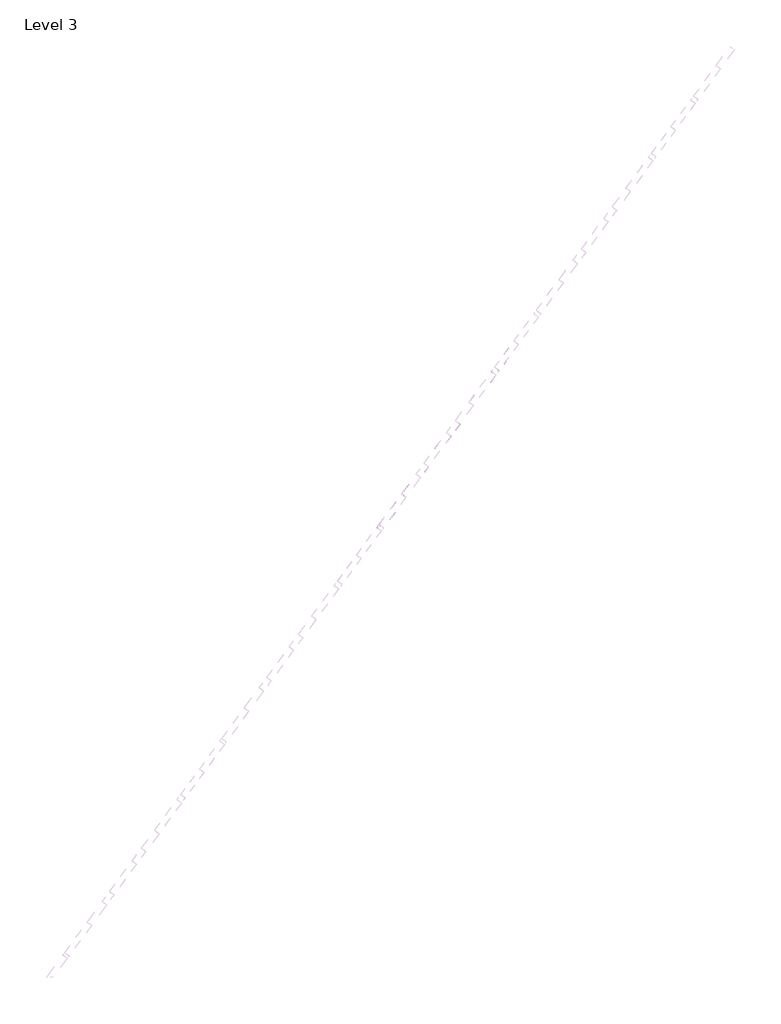
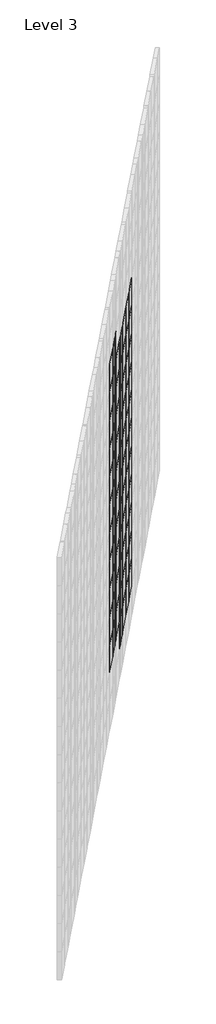
# One storey, part 7 of 9: 120 plates.
"""IFC4 building model written with IfcOpenShell, lengths in millimetres."""

import ifcopenshell
import ifcopenshell.guid

model = None  # the IFC model being written
_history = None  # IfcOwnerHistory: only IFC2X3 demands one
_inside = {}  # id of a spatial element -> (the spatial element, [elements in it])
_under = {}  # id of a project, library or spatial element -> (it, [spatial elements below it])
_declared = {}  # id of a project -> (the project, [libraries it declares])
_typed = {}  # id of a type object -> (the type object, [elements of that type])
_made_of = {}  # id of a material, layer set ... -> (it, [elements and type objects made of it])


def new_model(schema):
    """Start an empty IFC model of exactly this schema.

    Asked for "IFC4X3", IfcOpenShell would pick the latest addendum, in which some entities
    have other attributes; the version numbers below select the first issue.
    IFC2X3 requires an IfcOwnerHistory on every rooted entity: one is made here for all.
    """
    global model, _history
    if schema == "IFC4X3":
        model = ifcopenshell.file(schema_version=(4, 3, 0, 0))
    else:
        model = ifcopenshell.file(schema=schema)
    _inside.clear()
    _under.clear()
    _declared.clear()
    _typed.clear()
    _made_of.clear()
    _history = None
    if model.schema == "IFC2X3":
        org = make("IfcOrganization", Name="unknown")
        user = make(
            "IfcPersonAndOrganization",
            ThePerson=make("IfcPerson", FamilyName="unknown"),
            TheOrganization=org,
        )
        app = make(
            "IfcApplication",
            ApplicationDeveloper=org,
            Version="unknown",
            ApplicationFullName="unknown",
            ApplicationIdentifier="unknown",
        )
        _history = make(
            "IfcOwnerHistory",
            OwningUser=user,
            OwningApplication=app,
            ChangeAction="ADDED",
            CreationDate=0,
        )
    return model


def make(cls, **values):
    """One entity of the class cls with the attributes given. An attribute that is None is left unset."""
    return model.create_entity(
        cls, **{name: value for name, value in values.items() if value is not None}
    )


def rooted(cls, **values):
    """An entity with a GlobalId (a new one), such as an element, a storey or a relation."""
    return make(cls, GlobalId=ifcopenshell.guid.new(), OwnerHistory=_history, **values)


def si_unit(unit_type, name, prefix=None):
    """IfcSIUnit, for example si_unit("LENGTHUNIT", "METRE", prefix="MILLI")."""
    return make("IfcSIUnit", UnitType=unit_type, Prefix=prefix, Name=name)


def assignment(units):
    """IfcUnitAssignment: the units of a project."""
    return None if units is None else make("IfcUnitAssignment", Units=units)


def point(xyz):
    """IfcCartesianPoint."""
    return None if xyz is None else make("IfcCartesianPoint", Coordinates=xyz)


def direction(xyz):
    """IfcDirection."""
    return None if xyz is None else make("IfcDirection", DirectionRatios=xyz)


def frame(location, z_axis=None, x_axis=None):
    """IfcAxis2Placement3D, a coordinate frame: its origin and axes. An axis left out is left unset."""
    return make(
        "IfcAxis2Placement3D",
        Location=point(location),
        Axis=direction(z_axis),
        RefDirection=direction(x_axis),
    )


def origin():
    """The frame at (0, 0, 0) with its axes left unset."""
    return frame((0.0, 0.0, 0.0))


def origin_with_axes():
    """The frame at (0, 0, 0) with the z axis (0, 0, 1) and the x axis (1, 0, 0) written out."""
    return frame((0.0, 0.0, 0.0), z_axis=(0.0, 0.0, 1.0), x_axis=(1.0, 0.0, 0.0))


def place(relative_to, where):
    """IfcLocalPlacement: puts the frame where relative to a parent placement (None: the world)."""
    return make(
        "IfcLocalPlacement", PlacementRelTo=relative_to, RelativePlacement=where
    )


def context(
    kind, dimensions, precision=None, world=None, true_north=None, identifier=None
):
    """IfcGeometricRepresentationContext, for example the 3D "Model" context."""
    return make(
        "IfcGeometricRepresentationContext",
        ContextIdentifier=identifier,
        ContextType=kind,
        CoordinateSpaceDimension=dimensions,
        Precision=precision,
        WorldCoordinateSystem=world,
        TrueNorth=true_north,
    )


def project(units=None, contexts=None):
    """IfcProject with its units and contexts."""
    return rooted(
        "IfcProject",
        Name="project",
        RepresentationContexts=contexts,
        UnitsInContext=assignment(units),
    )


def spatial(cls, under=None, at=None, **own):
    """A site, building, storey or space (cls), placed at a placement, below another one or the project."""
    s = rooted(cls, ObjectPlacement=at, **own)
    if under is not None:
        _under.setdefault(under.id(), (under, []))[1].append(s)
    return s


def polyline(points):
    """IfcPolyline through the points."""
    return make("IfcPolyline", Points=[point(p) for p in points])


def outline(outer, holes=None, kind="AREA"):
    """IfcArbitraryClosedProfileDef: a profile drawn as a closed curve; with holes, ...WithVoids."""
    if holes is None:
        return make("IfcArbitraryClosedProfileDef", ProfileType=kind, OuterCurve=outer)
    return make(
        "IfcArbitraryProfileDefWithVoids",
        ProfileType=kind,
        OuterCurve=outer,
        InnerCurves=holes,
    )


def extrude(swept, where, along, depth):
    """IfcExtrudedAreaSolid: the profile swept, set in the frame where, extruded along a direction by depth."""
    return make(
        "IfcExtrudedAreaSolid",
        SweptArea=swept,
        Position=where,
        ExtrudedDirection=direction(along),
        Depth=depth,
    )


def shape(context_of_items, identifier, shape_type, items):
    """IfcShapeRepresentation: the items that make up one representation, for example the "Body"."""
    return make(
        "IfcShapeRepresentation",
        ContextOfItems=context_of_items,
        RepresentationIdentifier=identifier,
        RepresentationType=shape_type,
        Items=items,
    )


def source(mapping_origin, context_of_items, identifier, shape_type, items):
    """IfcRepresentationMap: a shape defined once, which mapped items show again and again."""
    return make(
        "IfcRepresentationMap",
        MappingOrigin=mapping_origin,
        MappedRepresentation=shape(context_of_items, identifier, shape_type, items),
    )


def transform(
    local_origin,
    x_axis=None,
    y_axis=None,
    z_axis=None,
    scale=None,
    scale2=None,
    scale3=None,
    uniform=True,
):
    """IfcCartesianTransformationOperator3D, or its non-uniform kind. x_axis, y_axis, z_axis: its Axis1, 2, 3."""
    if uniform:
        return make(
            "IfcCartesianTransformationOperator3D",
            Axis1=direction(x_axis),
            Axis2=direction(y_axis),
            LocalOrigin=point(local_origin),
            Scale=scale,
            Axis3=direction(z_axis),
        )
    return make(
        "IfcCartesianTransformationOperator3DnonUniform",
        Axis1=direction(x_axis),
        Axis2=direction(y_axis),
        LocalOrigin=point(local_origin),
        Scale=scale,
        Axis3=direction(z_axis),
        Scale2=scale2,
        Scale3=scale3,
    )


def mapped(mapping_source, mapping_target):
    """IfcMappedItem: shows the shape of a source again, moved by a transform."""
    return make(
        "IfcMappedItem", MappingSource=mapping_source, MappingTarget=mapping_target
    )


def made_of(thing, what):
    """Note that an element or type object is made of a material, layer set ...; save() writes the relation."""
    if what is not None:
        _made_of.setdefault(what.id(), (what, []))[1].append(thing)
    return thing


def element(
    cls,
    number,
    at=None,
    inside=None,
    cuts=None,
    type_object=None,
    material=None,
    context=None,
    identifier="Body",
    shape_type=None,
    held_by="IfcProductDefinitionShape",
    body=None,
    shapes=None,
    **own,
):
    """One element of the class cls, such as IfcWall. Its Tag is "e" and its number.

    at: its placement. inside: the storey or other place that contains it. cuts: it is an
    opening in that element (IfcRelVoidsElement). A single representation is given by context,
    identifier, shape_type and body (its items); several are given by shapes. held_by: the class
    of the entity that holds the representations. save() writes the other relations.
    """
    e = rooted(cls, Tag="e%d" % number, ObjectPlacement=at, **own)
    if body is not None:
        shapes = [shape(context, identifier, shape_type, body)]
    if shapes is not None:
        e.Representation = make(held_by, Representations=shapes)
    if inside is not None:
        _inside.setdefault(inside.id(), (inside, []))[1].append(e)
    if cuts is not None:
        rooted(
            "IfcRelVoidsElement", RelatingBuildingElement=cuts, RelatedOpeningElement=e
        )
    if type_object is not None:
        _typed.setdefault(type_object.id(), (type_object, []))[1].append(e)
    return made_of(e, material)


def aggregate(whole, parts):
    """IfcRelAggregates: a whole, such as a stair, and the parts it consists of."""
    return rooted("IfcRelAggregates", RelatingObject=whole, RelatedObjects=parts)


def save(model, path):
    """Write the relations noted so far, then the file.

    IfcRelAggregates (storeys below a building ...), IfcRelContainedInSpatialStructure (elements
    in a storey), IfcRelDefinesByType, IfcRelAssociatesMaterial and IfcRelDeclares: one each for
    every whole, place, type object, material and project.
    """
    for whole, parts in _under.values():
        aggregate(whole, parts)
    for where, things in _inside.values():
        rooted(
            "IfcRelContainedInSpatialStructure",
            RelatedElements=things,
            RelatingStructure=where,
        )
    for kind, things in _typed.values():
        rooted("IfcRelDefinesByType", RelatedObjects=things, RelatingType=kind)
    for what, things in _made_of.values():
        rooted("IfcRelAssociatesMaterial", RelatedObjects=things, RelatingMaterial=what)
    for by, libraries in _declared.values():
        rooted("IfcRelDeclares", RelatingContext=by, RelatedDefinitions=libraries)
    model.write(path)


def system_panel_glazed_b646d57f(model_context):
    return source(origin(), model_context, "Body", "SweptSolid", [
        extrude(outline(polyline([(8.5363468, 24.5), (-8.5363468, 24.5), (-8.5363468, 49.5), (8.5363468, 49.5), (8.5363468, 24.5)])), origin_with_axes(), (0.0, 0.0, 1.0), 200.0),
    ])


def system_panel_glazed_944c5575(model_context):
    return source(origin(), model_context, "Body", "SweptSolid", [
        extrude(outline(polyline([(30.0531077, 24.5), (-30.0531077, 24.5), (-30.0531077, 49.5), (30.0531077, 49.5), (30.0531077, 24.5)])), origin_with_axes(), (0.0, 0.0, 1.0), 200.0),
    ])


def system_panel_glazed_4b393385(model_context):
    return source(origin(), model_context, "Body", "SweptSolid", [
        extrude(outline(polyline([(51.5698685, 24.5), (-51.5698685, 24.5), (-51.5698685, 49.5), (51.5698685, 49.5), (51.5698685, 24.5)])), origin_with_axes(), (0.0, 0.0, 1.0), 200.0),
    ])


def system_panel_glazed_44cc28f0(model_context):
    return source(origin(), model_context, "Body", "SweptSolid", [
        extrude(outline(polyline([(73.0866293, 24.5), (-73.0866293, 24.5), (-73.0866293, 49.5), (73.0866293, 49.5), (73.0866293, 24.5)])), origin_with_axes(), (0.0, 0.0, 1.0), 200.0),
    ])


def system_panel_glazed_1ea8d406(model_context):
    return source(origin(), model_context, "Body", "SweptSolid", [
        extrude(outline(polyline([(85.0, 24.5), (-85.0, 24.5), (-85.0, 49.5), (85.0, 49.5), (85.0, 24.5)])), origin_with_axes(), (0.0, 0.0, 1.0), 200.0),
    ])


def system_panel_glazed_a6cffc9f(model_context):
    return source(origin(), model_context, "Body", "SweptSolid", [
        extrude(outline(polyline([(54.9468923, 24.5), (-54.9468923, 24.5), (-54.9468923, 49.5), (54.9468923, 49.5), (54.9468923, 24.5)])), origin_with_axes(), (0.0, 0.0, 1.0), 200.0),
    ])


def system_panel_glazed_52e3984b(model_context):
    return source(origin(), model_context, "Body", "SweptSolid", [
        extrude(outline(polyline([(33.4301315, 24.5), (-33.4301315, 24.5), (-33.4301315, 49.5), (33.4301315, 49.5), (33.4301315, 24.5)])), origin_with_axes(), (0.0, 0.0, 1.0), 200.0),
    ])


def system_panel_glazed_aeb916ba(model_context):
    return source(origin(), model_context, "Body", "SweptSolid", [
        extrude(outline(polyline([(11.9133707, 24.5), (-11.9133707, 24.5), (-11.9133707, 49.5), (11.9133707, 49.5), (11.9133707, 24.5)])), origin_with_axes(), (0.0, 0.0, 1.0), 200.0),
    ])


def system_panel_glazed_a3c9f580(model_context):
    return source(origin(), model_context, "Body", "SweptSolid", [
        extrude(outline(polyline([(75.3966098, 24.5), (-75.3966098, 24.5), (-75.3966098, 49.5), (75.3966098, 49.5), (75.3966098, 24.5)])), origin_with_axes(), (0.0, 0.0, 1.0), 200.0),
    ])


model = new_model("IFC4")

# Units and contexts
model_context = context("Model", 3, world=origin())
ifc_project = project(units=[si_unit("LENGTHUNIT", "METRE", prefix="MILLI")], contexts=[model_context])

# Site, building, storey
site = spatial("IfcSite", under=ifc_project)
building = spatial("IfcBuilding", under=site)
storey = spatial("IfcBuildingStorey", under=building, Name="Level 3", Elevation=22950.0)

# Plates
placement = place(None, origin())
system_panel_glazed_shape = system_panel_glazed_b646d57f(model_context)
element("IfcPlate", 1, ObjectType="System Panel : Glazed", at=placement, inside=storey, context=model_context, shape_type="MappedRepresentation", body=[
    mapped(system_panel_glazed_shape, transform((-31872.965562, 30068.174428, 35500.0), x_axis=(0.5920548138930122, 0.8058976965757569, 0.0), y_axis=(-0.8058976965757569, 0.5920548138930122, 0.0), z_axis=(0.0, 0.0, 1.0))),
])
element("IfcPlate", 2, ObjectType="System Panel : Glazed", at=placement, inside=storey, context=model_context, shape_type="MappedRepresentation", body=[
    mapped(system_panel_glazed_shape, transform((-31872.965562, 30068.174428, 35700.0), x_axis=(0.5920548138930122, 0.8058976965757569, 0.0), y_axis=(-0.8058976965757569, 0.5920548138930122, 0.0), z_axis=(0.0, 0.0, 1.0))),
])
element("IfcPlate", 3, ObjectType="System Panel : Glazed", at=placement, inside=storey, context=model_context, shape_type="MappedRepresentation", body=[
    mapped(system_panel_glazed_shape, transform((-31872.965562, 30068.174428, 35900.0), x_axis=(0.5920548138930122, 0.8058976965757569, 0.0), y_axis=(-0.8058976965757569, 0.5920548138930122, 0.0), z_axis=(0.0, 0.0, 1.0))),
])
element("IfcPlate", 4, ObjectType="System Panel : Glazed", at=placement, inside=storey, context=model_context, shape_type="MappedRepresentation", body=[
    mapped(system_panel_glazed_shape, transform((-31872.965562, 30068.174428, 36100.0), x_axis=(0.5920548138930122, 0.8058976965757569, 0.0), y_axis=(-0.8058976965757569, 0.5920548138930122, 0.0), z_axis=(0.0, 0.0, 1.0))),
])
element("IfcPlate", 5, ObjectType="System Panel : Glazed", at=placement, inside=storey, context=model_context, shape_type="MappedRepresentation", body=[
    mapped(system_panel_glazed_shape, transform((-31872.965562, 30068.174428, 36300.0), x_axis=(0.5920548138930122, 0.8058976965757569, 0.0), y_axis=(-0.8058976965757569, 0.5920548138930122, 0.0), z_axis=(0.0, 0.0, 1.0))),
])
element("IfcPlate", 6, ObjectType="System Panel : Glazed", at=placement, inside=storey, context=model_context, shape_type="MappedRepresentation", body=[
    mapped(system_panel_glazed_shape, transform((-31872.965562, 30068.174428, 36500.0), x_axis=(0.5920548138930122, 0.8058976965757569, 0.0), y_axis=(-0.8058976965757569, 0.5920548138930122, 0.0), z_axis=(0.0, 0.0, 1.0))),
])
element("IfcPlate", 7, ObjectType="System Panel : Glazed", at=placement, inside=storey, context=model_context, shape_type="MappedRepresentation", body=[
    mapped(system_panel_glazed_shape, transform((-31872.965562, 30068.174428, 36700.0), x_axis=(0.5920548138930122, 0.8058976965757569, 0.0), y_axis=(-0.8058976965757569, 0.5920548138930122, 0.0), z_axis=(0.0, 0.0, 1.0))),
])
element("IfcPlate", 8, ObjectType="System Panel : Glazed", at=placement, inside=storey, context=model_context, shape_type="MappedRepresentation", body=[
    mapped(system_panel_glazed_shape, transform((-31872.965562, 30068.174428, 36900.0), x_axis=(0.5920548138930122, 0.8058976965757569, 0.0), y_axis=(-0.8058976965757569, 0.5920548138930122, 0.0), z_axis=(0.0, 0.0, 1.0))),
])
element("IfcPlate", 9, ObjectType="System Panel : Glazed", at=placement, inside=storey, context=model_context, shape_type="MappedRepresentation", body=[
    mapped(system_panel_glazed_shape, transform((-31872.965562, 30068.174428, 37100.0), x_axis=(0.5920548138930122, 0.8058976965757569, 0.0), y_axis=(-0.8058976965757569, 0.5920548138930122, 0.0), z_axis=(0.0, 0.0, 1.0))),
])
element("IfcPlate", 10, ObjectType="System Panel : Glazed", at=placement, inside=storey, context=model_context, shape_type="MappedRepresentation", body=[
    mapped(system_panel_glazed_shape, transform((-31872.965562, 30068.174428, 37300.0), x_axis=(0.5920548138930122, 0.8058976965757569, 0.0), y_axis=(-0.8058976965757569, 0.5920548138930122, 0.0), z_axis=(0.0, 0.0, 1.0))),
])
element("IfcPlate", 11, ObjectType="System Panel : Glazed", at=placement, inside=storey, context=model_context, shape_type="MappedRepresentation", body=[
    mapped(system_panel_glazed_shape, transform((-31872.965562, 30068.174428, 37500.0), x_axis=(0.5920548138930122, 0.8058976965757569, 0.0), y_axis=(-0.8058976965757569, 0.5920548138930122, 0.0), z_axis=(0.0, 0.0, 1.0))),
])
system_panel_glazed_2_shape = system_panel_glazed_944c5575(model_context)
element("IfcPlate", 12, ObjectType="System Panel : Glazed", at=placement, inside=storey, context=model_context, shape_type="MappedRepresentation", body=[
    mapped(system_panel_glazed_2_shape, transform((-31684.4060271, 30324.8393368, 35500.0), x_axis=(0.5920548138930122, 0.8058976965757569, 0.0), y_axis=(-0.8058976965757569, 0.5920548138930122, 0.0), z_axis=(0.0, 0.0, 1.0))),
])
element("IfcPlate", 13, ObjectType="System Panel : Glazed", at=placement, inside=storey, context=model_context, shape_type="MappedRepresentation", body=[
    mapped(system_panel_glazed_2_shape, transform((-31684.4060271, 30324.8393368, 35700.0), x_axis=(0.5920548138930122, 0.8058976965757569, 0.0), y_axis=(-0.8058976965757569, 0.5920548138930122, 0.0), z_axis=(0.0, 0.0, 1.0))),
])
element("IfcPlate", 14, ObjectType="System Panel : Glazed", at=placement, inside=storey, context=model_context, shape_type="MappedRepresentation", body=[
    mapped(system_panel_glazed_2_shape, transform((-31684.4060271, 30324.8393368, 35900.0), x_axis=(0.5920548138930122, 0.8058976965757569, 0.0), y_axis=(-0.8058976965757569, 0.5920548138930122, 0.0), z_axis=(0.0, 0.0, 1.0))),
])
element("IfcPlate", 15, ObjectType="System Panel : Glazed", at=placement, inside=storey, context=model_context, shape_type="MappedRepresentation", body=[
    mapped(system_panel_glazed_2_shape, transform((-31684.4060271, 30324.8393368, 36100.0), x_axis=(0.5920548138930122, 0.8058976965757569, 0.0), y_axis=(-0.8058976965757569, 0.5920548138930122, 0.0), z_axis=(0.0, 0.0, 1.0))),
])
element("IfcPlate", 16, ObjectType="System Panel : Glazed", at=placement, inside=storey, context=model_context, shape_type="MappedRepresentation", body=[
    mapped(system_panel_glazed_2_shape, transform((-31684.4060271, 30324.8393368, 36300.0), x_axis=(0.5920548138930122, 0.8058976965757569, 0.0), y_axis=(-0.8058976965757569, 0.5920548138930122, 0.0), z_axis=(0.0, 0.0, 1.0))),
])
element("IfcPlate", 17, ObjectType="System Panel : Glazed", at=placement, inside=storey, context=model_context, shape_type="MappedRepresentation", body=[
    mapped(system_panel_glazed_2_shape, transform((-31684.4060271, 30324.8393368, 36500.0), x_axis=(0.5920548138930122, 0.8058976965757569, 0.0), y_axis=(-0.8058976965757569, 0.5920548138930122, 0.0), z_axis=(0.0, 0.0, 1.0))),
])
element("IfcPlate", 18, ObjectType="System Panel : Glazed", at=placement, inside=storey, context=model_context, shape_type="MappedRepresentation", body=[
    mapped(system_panel_glazed_2_shape, transform((-31684.4060271, 30324.8393368, 36700.0), x_axis=(0.5920548138930122, 0.8058976965757569, 0.0), y_axis=(-0.8058976965757569, 0.5920548138930122, 0.0), z_axis=(0.0, 0.0, 1.0))),
])
element("IfcPlate", 19, ObjectType="System Panel : Glazed", at=placement, inside=storey, context=model_context, shape_type="MappedRepresentation", body=[
    mapped(system_panel_glazed_2_shape, transform((-31684.4060271, 30324.8393368, 36900.0), x_axis=(0.5920548138930122, 0.8058976965757569, 0.0), y_axis=(-0.8058976965757569, 0.5920548138930122, 0.0), z_axis=(0.0, 0.0, 1.0))),
])
element("IfcPlate", 20, ObjectType="System Panel : Glazed", at=placement, inside=storey, context=model_context, shape_type="MappedRepresentation", body=[
    mapped(system_panel_glazed_2_shape, transform((-31684.4060271, 30324.8393368, 37100.0), x_axis=(0.5920548138930122, 0.8058976965757569, 0.0), y_axis=(-0.8058976965757569, 0.5920548138930122, 0.0), z_axis=(0.0, 0.0, 1.0))),
])
element("IfcPlate", 21, ObjectType="System Panel : Glazed", at=placement, inside=storey, context=model_context, shape_type="MappedRepresentation", body=[
    mapped(system_panel_glazed_2_shape, transform((-31684.4060271, 30324.8393368, 37300.0), x_axis=(0.5920548138930122, 0.8058976965757569, 0.0), y_axis=(-0.8058976965757569, 0.5920548138930122, 0.0), z_axis=(0.0, 0.0, 1.0))),
])
element("IfcPlate", 22, ObjectType="System Panel : Glazed", at=placement, inside=storey, context=model_context, shape_type="MappedRepresentation", body=[
    mapped(system_panel_glazed_2_shape, transform((-31684.4060271, 30324.8393368, 37500.0), x_axis=(0.5920548138930122, 0.8058976965757569, 0.0), y_axis=(-0.8058976965757569, 0.5920548138930122, 0.0), z_axis=(0.0, 0.0, 1.0))),
])
system_panel_glazed_3_shape = system_panel_glazed_4b393385(model_context)
element("IfcPlate", 23, ObjectType="System Panel : Glazed", at=placement, inside=storey, context=model_context, shape_type="MappedRepresentation", body=[
    mapped(system_panel_glazed_3_shape, transform((-31495.8464922, 30581.5042456, 35300.0), x_axis=(0.5920548138930122, 0.8058976965757569, 0.0), y_axis=(-0.8058976965757569, 0.5920548138930122, 0.0), z_axis=(0.0, 0.0, 1.0))),
])
element("IfcPlate", 24, ObjectType="System Panel : Glazed", at=placement, inside=storey, context=model_context, shape_type="MappedRepresentation", body=[
    mapped(system_panel_glazed_3_shape, transform((-31495.8464922, 30581.5042456, 35500.0), x_axis=(0.5920548138930122, 0.8058976965757569, 0.0), y_axis=(-0.8058976965757569, 0.5920548138930122, 0.0), z_axis=(0.0, 0.0, 1.0))),
])
element("IfcPlate", 25, ObjectType="System Panel : Glazed", at=placement, inside=storey, context=model_context, shape_type="MappedRepresentation", body=[
    mapped(system_panel_glazed_3_shape, transform((-31495.8464922, 30581.5042456, 35700.0), x_axis=(0.5920548138930122, 0.8058976965757569, 0.0), y_axis=(-0.8058976965757569, 0.5920548138930122, 0.0), z_axis=(0.0, 0.0, 1.0))),
])
element("IfcPlate", 26, ObjectType="System Panel : Glazed", at=placement, inside=storey, context=model_context, shape_type="MappedRepresentation", body=[
    mapped(system_panel_glazed_3_shape, transform((-31495.8464922, 30581.5042456, 35900.0), x_axis=(0.5920548138930122, 0.8058976965757569, 0.0), y_axis=(-0.8058976965757569, 0.5920548138930122, 0.0), z_axis=(0.0, 0.0, 1.0))),
])
element("IfcPlate", 27, ObjectType="System Panel : Glazed", at=placement, inside=storey, context=model_context, shape_type="MappedRepresentation", body=[
    mapped(system_panel_glazed_3_shape, transform((-31495.8464922, 30581.5042456, 36100.0), x_axis=(0.5920548138930122, 0.8058976965757569, 0.0), y_axis=(-0.8058976965757569, 0.5920548138930122, 0.0), z_axis=(0.0, 0.0, 1.0))),
])
element("IfcPlate", 28, ObjectType="System Panel : Glazed", at=placement, inside=storey, context=model_context, shape_type="MappedRepresentation", body=[
    mapped(system_panel_glazed_3_shape, transform((-31495.8464922, 30581.5042456, 36300.0), x_axis=(0.5920548138930122, 0.8058976965757569, 0.0), y_axis=(-0.8058976965757569, 0.5920548138930122, 0.0), z_axis=(0.0, 0.0, 1.0))),
])
element("IfcPlate", 29, ObjectType="System Panel : Glazed", at=placement, inside=storey, context=model_context, shape_type="MappedRepresentation", body=[
    mapped(system_panel_glazed_3_shape, transform((-31495.8464922, 30581.5042456, 36500.0), x_axis=(0.5920548138930122, 0.8058976965757569, 0.0), y_axis=(-0.8058976965757569, 0.5920548138930122, 0.0), z_axis=(0.0, 0.0, 1.0))),
])
element("IfcPlate", 30, ObjectType="System Panel : Glazed", at=placement, inside=storey, context=model_context, shape_type="MappedRepresentation", body=[
    mapped(system_panel_glazed_3_shape, transform((-31495.8464922, 30581.5042456, 36700.0), x_axis=(0.5920548138930122, 0.8058976965757569, 0.0), y_axis=(-0.8058976965757569, 0.5920548138930122, 0.0), z_axis=(0.0, 0.0, 1.0))),
])
element("IfcPlate", 31, ObjectType="System Panel : Glazed", at=placement, inside=storey, context=model_context, shape_type="MappedRepresentation", body=[
    mapped(system_panel_glazed_3_shape, transform((-31495.8464922, 30581.5042456, 36900.0), x_axis=(0.5920548138930122, 0.8058976965757569, 0.0), y_axis=(-0.8058976965757569, 0.5920548138930122, 0.0), z_axis=(0.0, 0.0, 1.0))),
])
element("IfcPlate", 32, ObjectType="System Panel : Glazed", at=placement, inside=storey, context=model_context, shape_type="MappedRepresentation", body=[
    mapped(system_panel_glazed_3_shape, transform((-31495.8464922, 30581.5042456, 37100.0), x_axis=(0.5920548138930122, 0.8058976965757569, 0.0), y_axis=(-0.8058976965757569, 0.5920548138930122, 0.0), z_axis=(0.0, 0.0, 1.0))),
])
element("IfcPlate", 33, ObjectType="System Panel : Glazed", at=placement, inside=storey, context=model_context, shape_type="MappedRepresentation", body=[
    mapped(system_panel_glazed_3_shape, transform((-31495.8464922, 30581.5042456, 37300.0), x_axis=(0.5920548138930122, 0.8058976965757569, 0.0), y_axis=(-0.8058976965757569, 0.5920548138930122, 0.0), z_axis=(0.0, 0.0, 1.0))),
])
system_panel_glazed_4_shape = system_panel_glazed_44cc28f0(model_context)
element("IfcPlate", 34, ObjectType="System Panel : Glazed", at=placement, inside=storey, context=model_context, shape_type="MappedRepresentation", body=[
    mapped(system_panel_glazed_4_shape, transform((-31307.2869573, 30838.1691545, 35300.0), x_axis=(0.5920548138930122, 0.8058976965757569, 0.0), y_axis=(-0.8058976965757569, 0.5920548138930122, 0.0), z_axis=(0.0, 0.0, 1.0))),
])
element("IfcPlate", 35, ObjectType="System Panel : Glazed", at=placement, inside=storey, context=model_context, shape_type="MappedRepresentation", body=[
    mapped(system_panel_glazed_4_shape, transform((-31307.2869573, 30838.1691545, 35500.0), x_axis=(0.5920548138930122, 0.8058976965757569, 0.0), y_axis=(-0.8058976965757569, 0.5920548138930122, 0.0), z_axis=(0.0, 0.0, 1.0))),
])
element("IfcPlate", 36, ObjectType="System Panel : Glazed", at=placement, inside=storey, context=model_context, shape_type="MappedRepresentation", body=[
    mapped(system_panel_glazed_4_shape, transform((-31307.2869573, 30838.1691545, 35700.0), x_axis=(0.5920548138930122, 0.8058976965757569, 0.0), y_axis=(-0.8058976965757569, 0.5920548138930122, 0.0), z_axis=(0.0, 0.0, 1.0))),
])
element("IfcPlate", 37, ObjectType="System Panel : Glazed", at=placement, inside=storey, context=model_context, shape_type="MappedRepresentation", body=[
    mapped(system_panel_glazed_4_shape, transform((-31307.2869573, 30838.1691545, 35900.0), x_axis=(0.5920548138930122, 0.8058976965757569, 0.0), y_axis=(-0.8058976965757569, 0.5920548138930122, 0.0), z_axis=(0.0, 0.0, 1.0))),
])
element("IfcPlate", 38, ObjectType="System Panel : Glazed", at=placement, inside=storey, context=model_context, shape_type="MappedRepresentation", body=[
    mapped(system_panel_glazed_4_shape, transform((-31307.2869573, 30838.1691545, 36100.0), x_axis=(0.5920548138930122, 0.8058976965757569, 0.0), y_axis=(-0.8058976965757569, 0.5920548138930122, 0.0), z_axis=(0.0, 0.0, 1.0))),
])
element("IfcPlate", 39, ObjectType="System Panel : Glazed", at=placement, inside=storey, context=model_context, shape_type="MappedRepresentation", body=[
    mapped(system_panel_glazed_4_shape, transform((-31307.2869573, 30838.1691545, 36300.0), x_axis=(0.5920548138930122, 0.8058976965757569, 0.0), y_axis=(-0.8058976965757569, 0.5920548138930122, 0.0), z_axis=(0.0, 0.0, 1.0))),
])
element("IfcPlate", 40, ObjectType="System Panel : Glazed", at=placement, inside=storey, context=model_context, shape_type="MappedRepresentation", body=[
    mapped(system_panel_glazed_4_shape, transform((-31307.2869573, 30838.1691545, 36500.0), x_axis=(0.5920548138930122, 0.8058976965757569, 0.0), y_axis=(-0.8058976965757569, 0.5920548138930122, 0.0), z_axis=(0.0, 0.0, 1.0))),
])
element("IfcPlate", 41, ObjectType="System Panel : Glazed", at=placement, inside=storey, context=model_context, shape_type="MappedRepresentation", body=[
    mapped(system_panel_glazed_4_shape, transform((-31307.2869573, 30838.1691545, 36700.0), x_axis=(0.5920548138930122, 0.8058976965757569, 0.0), y_axis=(-0.8058976965757569, 0.5920548138930122, 0.0), z_axis=(0.0, 0.0, 1.0))),
])
element("IfcPlate", 42, ObjectType="System Panel : Glazed", at=placement, inside=storey, context=model_context, shape_type="MappedRepresentation", body=[
    mapped(system_panel_glazed_4_shape, transform((-31307.2869573, 30838.1691545, 36900.0), x_axis=(0.5920548138930122, 0.8058976965757569, 0.0), y_axis=(-0.8058976965757569, 0.5920548138930122, 0.0), z_axis=(0.0, 0.0, 1.0))),
])
element("IfcPlate", 43, ObjectType="System Panel : Glazed", at=placement, inside=storey, context=model_context, shape_type="MappedRepresentation", body=[
    mapped(system_panel_glazed_4_shape, transform((-31307.2869573, 30838.1691545, 37100.0), x_axis=(0.5920548138930122, 0.8058976965757569, 0.0), y_axis=(-0.8058976965757569, 0.5920548138930122, 0.0), z_axis=(0.0, 0.0, 1.0))),
])
element("IfcPlate", 44, ObjectType="System Panel : Glazed", at=placement, inside=storey, context=model_context, shape_type="MappedRepresentation", body=[
    mapped(system_panel_glazed_4_shape, transform((-31307.2869573, 30838.1691545, 37300.0), x_axis=(0.5920548138930122, 0.8058976965757569, 0.0), y_axis=(-0.8058976965757569, 0.5920548138930122, 0.0), z_axis=(0.0, 0.0, 1.0))),
])
system_panel_glazed_5_shape = system_panel_glazed_1ea8d406(model_context)
element("IfcPlate", 45, ObjectType="System Panel : Glazed", at=placement, inside=storey, context=model_context, shape_type="MappedRepresentation", body=[
    mapped(system_panel_glazed_5_shape, transform((-31414.9896441, 30691.5655881, 35300.0), x_axis=(0.5920548138930122, 0.8058976965757569, 0.0), y_axis=(-0.8058976965757569, 0.5920548138930122, 0.0), z_axis=(0.0, 0.0, 1.0))),
])
element("IfcPlate", 46, ObjectType="System Panel : Glazed", at=placement, inside=storey, context=model_context, shape_type="MappedRepresentation", body=[
    mapped(system_panel_glazed_5_shape, transform((-31817.5869176, 30143.5551544, 35500.0), x_axis=(0.5920548138930122, 0.8058976965757569, 0.0), y_axis=(-0.8058976965757569, 0.5920548138930122, 0.0), z_axis=(0.0, 0.0, 1.0))),
])
element("IfcPlate", 47, ObjectType="System Panel : Glazed", at=placement, inside=storey, context=model_context, shape_type="MappedRepresentation", body=[
    mapped(system_panel_glazed_5_shape, transform((-31616.2882809, 30417.5603713, 35500.0), x_axis=(0.5920548138930122, 0.8058976965757569, 0.0), y_axis=(-0.8058976965757569, 0.5920548138930122, 0.0), z_axis=(0.0, 0.0, 1.0))),
])
element("IfcPlate", 48, ObjectType="System Panel : Glazed", at=placement, inside=storey, context=model_context, shape_type="MappedRepresentation", body=[
    mapped(system_panel_glazed_5_shape, transform((-31414.9896441, 30691.5655881, 35500.0), x_axis=(0.5920548138930122, 0.8058976965757569, 0.0), y_axis=(-0.8058976965757569, 0.5920548138930122, 0.0), z_axis=(0.0, 0.0, 1.0))),
])
element("IfcPlate", 49, ObjectType="System Panel : Glazed", at=placement, inside=storey, context=model_context, shape_type="MappedRepresentation", body=[
    mapped(system_panel_glazed_5_shape, transform((-31817.5869176, 30143.5551544, 35700.0), x_axis=(0.5920548138930122, 0.8058976965757569, 0.0), y_axis=(-0.8058976965757569, 0.5920548138930122, 0.0), z_axis=(0.0, 0.0, 1.0))),
])
element("IfcPlate", 50, ObjectType="System Panel : Glazed", at=placement, inside=storey, context=model_context, shape_type="MappedRepresentation", body=[
    mapped(system_panel_glazed_5_shape, transform((-31616.2882809, 30417.5603713, 35700.0), x_axis=(0.5920548138930122, 0.8058976965757569, 0.0), y_axis=(-0.8058976965757569, 0.5920548138930122, 0.0), z_axis=(0.0, 0.0, 1.0))),
])
element("IfcPlate", 51, ObjectType="System Panel : Glazed", at=placement, inside=storey, context=model_context, shape_type="MappedRepresentation", body=[
    mapped(system_panel_glazed_5_shape, transform((-31414.9896441, 30691.5655881, 35700.0), x_axis=(0.5920548138930122, 0.8058976965757569, 0.0), y_axis=(-0.8058976965757569, 0.5920548138930122, 0.0), z_axis=(0.0, 0.0, 1.0))),
])
element("IfcPlate", 52, ObjectType="System Panel : Glazed", at=placement, inside=storey, context=model_context, shape_type="MappedRepresentation", body=[
    mapped(system_panel_glazed_5_shape, transform((-31817.5869176, 30143.5551544, 35900.0), x_axis=(0.5920548138930122, 0.8058976965757569, 0.0), y_axis=(-0.8058976965757569, 0.5920548138930122, 0.0), z_axis=(0.0, 0.0, 1.0))),
])
element("IfcPlate", 53, ObjectType="System Panel : Glazed", at=placement, inside=storey, context=model_context, shape_type="MappedRepresentation", body=[
    mapped(system_panel_glazed_5_shape, transform((-31616.2882809, 30417.5603713, 35900.0), x_axis=(0.5920548138930122, 0.8058976965757569, 0.0), y_axis=(-0.8058976965757569, 0.5920548138930122, 0.0), z_axis=(0.0, 0.0, 1.0))),
])
element("IfcPlate", 54, ObjectType="System Panel : Glazed", at=placement, inside=storey, context=model_context, shape_type="MappedRepresentation", body=[
    mapped(system_panel_glazed_5_shape, transform((-31414.9896441, 30691.5655881, 35900.0), x_axis=(0.5920548138930122, 0.8058976965757569, 0.0), y_axis=(-0.8058976965757569, 0.5920548138930122, 0.0), z_axis=(0.0, 0.0, 1.0))),
])
element("IfcPlate", 55, ObjectType="System Panel : Glazed", at=placement, inside=storey, context=model_context, shape_type="MappedRepresentation", body=[
    mapped(system_panel_glazed_5_shape, transform((-31817.5869176, 30143.5551544, 36100.0), x_axis=(0.5920548138930122, 0.8058976965757569, 0.0), y_axis=(-0.8058976965757569, 0.5920548138930122, 0.0), z_axis=(0.0, 0.0, 1.0))),
])
element("IfcPlate", 56, ObjectType="System Panel : Glazed", at=placement, inside=storey, context=model_context, shape_type="MappedRepresentation", body=[
    mapped(system_panel_glazed_5_shape, transform((-31616.2882809, 30417.5603713, 36100.0), x_axis=(0.5920548138930122, 0.8058976965757569, 0.0), y_axis=(-0.8058976965757569, 0.5920548138930122, 0.0), z_axis=(0.0, 0.0, 1.0))),
])
element("IfcPlate", 57, ObjectType="System Panel : Glazed", at=placement, inside=storey, context=model_context, shape_type="MappedRepresentation", body=[
    mapped(system_panel_glazed_5_shape, transform((-31414.9896441, 30691.5655881, 36100.0), x_axis=(0.5920548138930122, 0.8058976965757569, 0.0), y_axis=(-0.8058976965757569, 0.5920548138930122, 0.0), z_axis=(0.0, 0.0, 1.0))),
])
element("IfcPlate", 58, ObjectType="System Panel : Glazed", at=placement, inside=storey, context=model_context, shape_type="MappedRepresentation", body=[
    mapped(system_panel_glazed_5_shape, transform((-31817.5869176, 30143.5551544, 36300.0), x_axis=(0.5920548138930122, 0.8058976965757569, 0.0), y_axis=(-0.8058976965757569, 0.5920548138930122, 0.0), z_axis=(0.0, 0.0, 1.0))),
])
element("IfcPlate", 59, ObjectType="System Panel : Glazed", at=placement, inside=storey, context=model_context, shape_type="MappedRepresentation", body=[
    mapped(system_panel_glazed_5_shape, transform((-31616.2882809, 30417.5603713, 36300.0), x_axis=(0.5920548138930122, 0.8058976965757569, 0.0), y_axis=(-0.8058976965757569, 0.5920548138930122, 0.0), z_axis=(0.0, 0.0, 1.0))),
])
element("IfcPlate", 60, ObjectType="System Panel : Glazed", at=placement, inside=storey, context=model_context, shape_type="MappedRepresentation", body=[
    mapped(system_panel_glazed_5_shape, transform((-31414.9896441, 30691.5655881, 36300.0), x_axis=(0.5920548138930122, 0.8058976965757569, 0.0), y_axis=(-0.8058976965757569, 0.5920548138930122, 0.0), z_axis=(0.0, 0.0, 1.0))),
])
element("IfcPlate", 61, ObjectType="System Panel : Glazed", at=placement, inside=storey, context=model_context, shape_type="MappedRepresentation", body=[
    mapped(system_panel_glazed_5_shape, transform((-31817.5869176, 30143.5551544, 36500.0), x_axis=(0.5920548138930122, 0.8058976965757569, 0.0), y_axis=(-0.8058976965757569, 0.5920548138930122, 0.0), z_axis=(0.0, 0.0, 1.0))),
])
element("IfcPlate", 62, ObjectType="System Panel : Glazed", at=placement, inside=storey, context=model_context, shape_type="MappedRepresentation", body=[
    mapped(system_panel_glazed_5_shape, transform((-31616.2882809, 30417.5603713, 36500.0), x_axis=(0.5920548138930122, 0.8058976965757569, 0.0), y_axis=(-0.8058976965757569, 0.5920548138930122, 0.0), z_axis=(0.0, 0.0, 1.0))),
])
element("IfcPlate", 63, ObjectType="System Panel : Glazed", at=placement, inside=storey, context=model_context, shape_type="MappedRepresentation", body=[
    mapped(system_panel_glazed_5_shape, transform((-31414.9896441, 30691.5655881, 36500.0), x_axis=(0.5920548138930122, 0.8058976965757569, 0.0), y_axis=(-0.8058976965757569, 0.5920548138930122, 0.0), z_axis=(0.0, 0.0, 1.0))),
])
element("IfcPlate", 64, ObjectType="System Panel : Glazed", at=placement, inside=storey, context=model_context, shape_type="MappedRepresentation", body=[
    mapped(system_panel_glazed_5_shape, transform((-31817.5869176, 30143.5551544, 36700.0), x_axis=(0.5920548138930122, 0.8058976965757569, 0.0), y_axis=(-0.8058976965757569, 0.5920548138930122, 0.0), z_axis=(0.0, 0.0, 1.0))),
])
element("IfcPlate", 65, ObjectType="System Panel : Glazed", at=placement, inside=storey, context=model_context, shape_type="MappedRepresentation", body=[
    mapped(system_panel_glazed_5_shape, transform((-31616.2882809, 30417.5603713, 36700.0), x_axis=(0.5920548138930122, 0.8058976965757569, 0.0), y_axis=(-0.8058976965757569, 0.5920548138930122, 0.0), z_axis=(0.0, 0.0, 1.0))),
])
element("IfcPlate", 66, ObjectType="System Panel : Glazed", at=placement, inside=storey, context=model_context, shape_type="MappedRepresentation", body=[
    mapped(system_panel_glazed_5_shape, transform((-31414.9896441, 30691.5655881, 36700.0), x_axis=(0.5920548138930122, 0.8058976965757569, 0.0), y_axis=(-0.8058976965757569, 0.5920548138930122, 0.0), z_axis=(0.0, 0.0, 1.0))),
])
element("IfcPlate", 67, ObjectType="System Panel : Glazed", at=placement, inside=storey, context=model_context, shape_type="MappedRepresentation", body=[
    mapped(system_panel_glazed_5_shape, transform((-31817.5869176, 30143.5551544, 36900.0), x_axis=(0.5920548138930122, 0.8058976965757569, 0.0), y_axis=(-0.8058976965757569, 0.5920548138930122, 0.0), z_axis=(0.0, 0.0, 1.0))),
])
element("IfcPlate", 68, ObjectType="System Panel : Glazed", at=placement, inside=storey, context=model_context, shape_type="MappedRepresentation", body=[
    mapped(system_panel_glazed_5_shape, transform((-31616.2882809, 30417.5603713, 36900.0), x_axis=(0.5920548138930122, 0.8058976965757569, 0.0), y_axis=(-0.8058976965757569, 0.5920548138930122, 0.0), z_axis=(0.0, 0.0, 1.0))),
])
element("IfcPlate", 69, ObjectType="System Panel : Glazed", at=placement, inside=storey, context=model_context, shape_type="MappedRepresentation", body=[
    mapped(system_panel_glazed_5_shape, transform((-31414.9896441, 30691.5655881, 36900.0), x_axis=(0.5920548138930122, 0.8058976965757569, 0.0), y_axis=(-0.8058976965757569, 0.5920548138930122, 0.0), z_axis=(0.0, 0.0, 1.0))),
])
element("IfcPlate", 70, ObjectType="System Panel : Glazed", at=placement, inside=storey, context=model_context, shape_type="MappedRepresentation", body=[
    mapped(system_panel_glazed_5_shape, transform((-31817.5869176, 30143.5551544, 37100.0), x_axis=(0.5920548138930122, 0.8058976965757569, 0.0), y_axis=(-0.8058976965757569, 0.5920548138930122, 0.0), z_axis=(0.0, 0.0, 1.0))),
])
element("IfcPlate", 71, ObjectType="System Panel : Glazed", at=placement, inside=storey, context=model_context, shape_type="MappedRepresentation", body=[
    mapped(system_panel_glazed_5_shape, transform((-31616.2882809, 30417.5603713, 37100.0), x_axis=(0.5920548138930122, 0.8058976965757569, 0.0), y_axis=(-0.8058976965757569, 0.5920548138930122, 0.0), z_axis=(0.0, 0.0, 1.0))),
])
element("IfcPlate", 72, ObjectType="System Panel : Glazed", at=placement, inside=storey, context=model_context, shape_type="MappedRepresentation", body=[
    mapped(system_panel_glazed_5_shape, transform((-31414.9896441, 30691.5655881, 37100.0), x_axis=(0.5920548138930122, 0.8058976965757569, 0.0), y_axis=(-0.8058976965757569, 0.5920548138930122, 0.0), z_axis=(0.0, 0.0, 1.0))),
])
element("IfcPlate", 73, ObjectType="System Panel : Glazed", at=placement, inside=storey, context=model_context, shape_type="MappedRepresentation", body=[
    mapped(system_panel_glazed_5_shape, transform((-31817.5869176, 30143.5551544, 37300.0), x_axis=(0.5920548138930122, 0.8058976965757569, 0.0), y_axis=(-0.8058976965757569, 0.5920548138930122, 0.0), z_axis=(0.0, 0.0, 1.0))),
])
element("IfcPlate", 74, ObjectType="System Panel : Glazed", at=placement, inside=storey, context=model_context, shape_type="MappedRepresentation", body=[
    mapped(system_panel_glazed_5_shape, transform((-31616.2882809, 30417.5603713, 37300.0), x_axis=(0.5920548138930122, 0.8058976965757569, 0.0), y_axis=(-0.8058976965757569, 0.5920548138930122, 0.0), z_axis=(0.0, 0.0, 1.0))),
])
element("IfcPlate", 75, ObjectType="System Panel : Glazed", at=placement, inside=storey, context=model_context, shape_type="MappedRepresentation", body=[
    mapped(system_panel_glazed_5_shape, transform((-31414.9896441, 30691.5655881, 37300.0), x_axis=(0.5920548138930122, 0.8058976965757569, 0.0), y_axis=(-0.8058976965757569, 0.5920548138930122, 0.0), z_axis=(0.0, 0.0, 1.0))),
])
element("IfcPlate", 76, ObjectType="System Panel : Glazed", at=placement, inside=storey, context=model_context, shape_type="MappedRepresentation", body=[
    mapped(system_panel_glazed_5_shape, transform((-31817.5869176, 30143.5551544, 37500.0), x_axis=(0.5920548138930122, 0.8058976965757569, 0.0), y_axis=(-0.8058976965757569, 0.5920548138930122, 0.0), z_axis=(0.0, 0.0, 1.0))),
])
system_panel_glazed_6_shape = system_panel_glazed_a6cffc9f(model_context)
element("IfcPlate", 77, ObjectType="System Panel : Glazed", at=placement, inside=storey, context=model_context, shape_type="MappedRepresentation", body=[
    mapped(system_panel_glazed_6_shape, transform((-31734.7306863, 30256.3380326, 35500.0), x_axis=(0.5920548138930122, 0.8058976965757569, 0.0), y_axis=(-0.8058976965757569, 0.5920548138930122, 0.0), z_axis=(0.0, 0.0, 1.0))),
])
element("IfcPlate", 78, ObjectType="System Panel : Glazed", at=placement, inside=storey, context=model_context, shape_type="MappedRepresentation", body=[
    mapped(system_panel_glazed_6_shape, transform((-31734.7306863, 30256.3380326, 35700.0), x_axis=(0.5920548138930122, 0.8058976965757569, 0.0), y_axis=(-0.8058976965757569, 0.5920548138930122, 0.0), z_axis=(0.0, 0.0, 1.0))),
])
element("IfcPlate", 79, ObjectType="System Panel : Glazed", at=placement, inside=storey, context=model_context, shape_type="MappedRepresentation", body=[
    mapped(system_panel_glazed_6_shape, transform((-31734.7306863, 30256.3380326, 35900.0), x_axis=(0.5920548138930122, 0.8058976965757569, 0.0), y_axis=(-0.8058976965757569, 0.5920548138930122, 0.0), z_axis=(0.0, 0.0, 1.0))),
])
element("IfcPlate", 80, ObjectType="System Panel : Glazed", at=placement, inside=storey, context=model_context, shape_type="MappedRepresentation", body=[
    mapped(system_panel_glazed_6_shape, transform((-31734.7306863, 30256.3380326, 36100.0), x_axis=(0.5920548138930122, 0.8058976965757569, 0.0), y_axis=(-0.8058976965757569, 0.5920548138930122, 0.0), z_axis=(0.0, 0.0, 1.0))),
])
element("IfcPlate", 81, ObjectType="System Panel : Glazed", at=placement, inside=storey, context=model_context, shape_type="MappedRepresentation", body=[
    mapped(system_panel_glazed_6_shape, transform((-31734.7306863, 30256.3380326, 36300.0), x_axis=(0.5920548138930122, 0.8058976965757569, 0.0), y_axis=(-0.8058976965757569, 0.5920548138930122, 0.0), z_axis=(0.0, 0.0, 1.0))),
])
element("IfcPlate", 82, ObjectType="System Panel : Glazed", at=placement, inside=storey, context=model_context, shape_type="MappedRepresentation", body=[
    mapped(system_panel_glazed_6_shape, transform((-31734.7306863, 30256.3380326, 36500.0), x_axis=(0.5920548138930122, 0.8058976965757569, 0.0), y_axis=(-0.8058976965757569, 0.5920548138930122, 0.0), z_axis=(0.0, 0.0, 1.0))),
])
element("IfcPlate", 83, ObjectType="System Panel : Glazed", at=placement, inside=storey, context=model_context, shape_type="MappedRepresentation", body=[
    mapped(system_panel_glazed_6_shape, transform((-31734.7306863, 30256.3380326, 36700.0), x_axis=(0.5920548138930122, 0.8058976965757569, 0.0), y_axis=(-0.8058976965757569, 0.5920548138930122, 0.0), z_axis=(0.0, 0.0, 1.0))),
])
element("IfcPlate", 84, ObjectType="System Panel : Glazed", at=placement, inside=storey, context=model_context, shape_type="MappedRepresentation", body=[
    mapped(system_panel_glazed_6_shape, transform((-31734.7306863, 30256.3380326, 36900.0), x_axis=(0.5920548138930122, 0.8058976965757569, 0.0), y_axis=(-0.8058976965757569, 0.5920548138930122, 0.0), z_axis=(0.0, 0.0, 1.0))),
])
element("IfcPlate", 85, ObjectType="System Panel : Glazed", at=placement, inside=storey, context=model_context, shape_type="MappedRepresentation", body=[
    mapped(system_panel_glazed_6_shape, transform((-31734.7306863, 30256.3380326, 37100.0), x_axis=(0.5920548138930122, 0.8058976965757569, 0.0), y_axis=(-0.8058976965757569, 0.5920548138930122, 0.0), z_axis=(0.0, 0.0, 1.0))),
])
element("IfcPlate", 86, ObjectType="System Panel : Glazed", at=placement, inside=storey, context=model_context, shape_type="MappedRepresentation", body=[
    mapped(system_panel_glazed_6_shape, transform((-31734.7306863, 30256.3380326, 37300.0), x_axis=(0.5920548138930122, 0.8058976965757569, 0.0), y_axis=(-0.8058976965757569, 0.5920548138930122, 0.0), z_axis=(0.0, 0.0, 1.0))),
])
element("IfcPlate", 87, ObjectType="System Panel : Glazed", at=placement, inside=storey, context=model_context, shape_type="MappedRepresentation", body=[
    mapped(system_panel_glazed_6_shape, transform((-31734.7306863, 30256.3380326, 37500.0), x_axis=(0.5920548138930122, 0.8058976965757569, 0.0), y_axis=(-0.8058976965757569, 0.5920548138930122, 0.0), z_axis=(0.0, 0.0, 1.0))),
])
system_panel_glazed_7_shape = system_panel_glazed_52e3984b(model_context)
element("IfcPlate", 88, ObjectType="System Panel : Glazed", at=placement, inside=storey, context=model_context, shape_type="MappedRepresentation", body=[
    mapped(system_panel_glazed_7_shape, transform((-31546.1711514, 30513.0029414, 35300.0), x_axis=(0.5920548138930122, 0.8058976965757569, 0.0), y_axis=(-0.8058976965757569, 0.5920548138930122, 0.0), z_axis=(0.0, 0.0, 1.0))),
])
element("IfcPlate", 89, ObjectType="System Panel : Glazed", at=placement, inside=storey, context=model_context, shape_type="MappedRepresentation", body=[
    mapped(system_panel_glazed_7_shape, transform((-31546.1711514, 30513.0029414, 35500.0), x_axis=(0.5920548138930122, 0.8058976965757569, 0.0), y_axis=(-0.8058976965757569, 0.5920548138930122, 0.0), z_axis=(0.0, 0.0, 1.0))),
])
element("IfcPlate", 90, ObjectType="System Panel : Glazed", at=placement, inside=storey, context=model_context, shape_type="MappedRepresentation", body=[
    mapped(system_panel_glazed_7_shape, transform((-31546.1711514, 30513.0029414, 35700.0), x_axis=(0.5920548138930122, 0.8058976965757569, 0.0), y_axis=(-0.8058976965757569, 0.5920548138930122, 0.0), z_axis=(0.0, 0.0, 1.0))),
])
element("IfcPlate", 91, ObjectType="System Panel : Glazed", at=placement, inside=storey, context=model_context, shape_type="MappedRepresentation", body=[
    mapped(system_panel_glazed_7_shape, transform((-31546.1711514, 30513.0029414, 35900.0), x_axis=(0.5920548138930122, 0.8058976965757569, 0.0), y_axis=(-0.8058976965757569, 0.5920548138930122, 0.0), z_axis=(0.0, 0.0, 1.0))),
])
element("IfcPlate", 92, ObjectType="System Panel : Glazed", at=placement, inside=storey, context=model_context, shape_type="MappedRepresentation", body=[
    mapped(system_panel_glazed_7_shape, transform((-31546.1711514, 30513.0029414, 36100.0), x_axis=(0.5920548138930122, 0.8058976965757569, 0.0), y_axis=(-0.8058976965757569, 0.5920548138930122, 0.0), z_axis=(0.0, 0.0, 1.0))),
])
element("IfcPlate", 93, ObjectType="System Panel : Glazed", at=placement, inside=storey, context=model_context, shape_type="MappedRepresentation", body=[
    mapped(system_panel_glazed_7_shape, transform((-31546.1711514, 30513.0029414, 36300.0), x_axis=(0.5920548138930122, 0.8058976965757569, 0.0), y_axis=(-0.8058976965757569, 0.5920548138930122, 0.0), z_axis=(0.0, 0.0, 1.0))),
])
element("IfcPlate", 94, ObjectType="System Panel : Glazed", at=placement, inside=storey, context=model_context, shape_type="MappedRepresentation", body=[
    mapped(system_panel_glazed_7_shape, transform((-31546.1711514, 30513.0029414, 36500.0), x_axis=(0.5920548138930122, 0.8058976965757569, 0.0), y_axis=(-0.8058976965757569, 0.5920548138930122, 0.0), z_axis=(0.0, 0.0, 1.0))),
])
element("IfcPlate", 95, ObjectType="System Panel : Glazed", at=placement, inside=storey, context=model_context, shape_type="MappedRepresentation", body=[
    mapped(system_panel_glazed_7_shape, transform((-31546.1711514, 30513.0029414, 36700.0), x_axis=(0.5920548138930122, 0.8058976965757569, 0.0), y_axis=(-0.8058976965757569, 0.5920548138930122, 0.0), z_axis=(0.0, 0.0, 1.0))),
])
element("IfcPlate", 96, ObjectType="System Panel : Glazed", at=placement, inside=storey, context=model_context, shape_type="MappedRepresentation", body=[
    mapped(system_panel_glazed_7_shape, transform((-31546.1711514, 30513.0029414, 36900.0), x_axis=(0.5920548138930122, 0.8058976965757569, 0.0), y_axis=(-0.8058976965757569, 0.5920548138930122, 0.0), z_axis=(0.0, 0.0, 1.0))),
])
element("IfcPlate", 97, ObjectType="System Panel : Glazed", at=placement, inside=storey, context=model_context, shape_type="MappedRepresentation", body=[
    mapped(system_panel_glazed_7_shape, transform((-31546.1711514, 30513.0029414, 37100.0), x_axis=(0.5920548138930122, 0.8058976965757569, 0.0), y_axis=(-0.8058976965757569, 0.5920548138930122, 0.0), z_axis=(0.0, 0.0, 1.0))),
])
element("IfcPlate", 98, ObjectType="System Panel : Glazed", at=placement, inside=storey, context=model_context, shape_type="MappedRepresentation", body=[
    mapped(system_panel_glazed_7_shape, transform((-31546.1711514, 30513.0029414, 37300.0), x_axis=(0.5920548138930122, 0.8058976965757569, 0.0), y_axis=(-0.8058976965757569, 0.5920548138930122, 0.0), z_axis=(0.0, 0.0, 1.0))),
])
system_panel_glazed_8_shape = system_panel_glazed_aeb916ba(model_context)
element("IfcPlate", 99, ObjectType="System Panel : Glazed", at=placement, inside=storey, context=model_context, shape_type="MappedRepresentation", body=[
    mapped(system_panel_glazed_8_shape, transform((-31357.6116165, 30769.6678503, 35300.0), x_axis=(0.5920548138930122, 0.8058976965757569, 0.0), y_axis=(-0.8058976965757569, 0.5920548138930122, 0.0), z_axis=(0.0, 0.0, 1.0))),
])
element("IfcPlate", 100, ObjectType="System Panel : Glazed", at=placement, inside=storey, context=model_context, shape_type="MappedRepresentation", body=[
    mapped(system_panel_glazed_8_shape, transform((-31357.6116165, 30769.6678503, 35500.0), x_axis=(0.5920548138930122, 0.8058976965757569, 0.0), y_axis=(-0.8058976965757569, 0.5920548138930122, 0.0), z_axis=(0.0, 0.0, 1.0))),
])
element("IfcPlate", 101, ObjectType="System Panel : Glazed", at=placement, inside=storey, context=model_context, shape_type="MappedRepresentation", body=[
    mapped(system_panel_glazed_8_shape, transform((-31357.6116165, 30769.6678503, 35700.0), x_axis=(0.5920548138930122, 0.8058976965757569, 0.0), y_axis=(-0.8058976965757569, 0.5920548138930122, 0.0), z_axis=(0.0, 0.0, 1.0))),
])
element("IfcPlate", 102, ObjectType="System Panel : Glazed", at=placement, inside=storey, context=model_context, shape_type="MappedRepresentation", body=[
    mapped(system_panel_glazed_8_shape, transform((-31357.6116165, 30769.6678503, 35900.0), x_axis=(0.5920548138930122, 0.8058976965757569, 0.0), y_axis=(-0.8058976965757569, 0.5920548138930122, 0.0), z_axis=(0.0, 0.0, 1.0))),
])
element("IfcPlate", 103, ObjectType="System Panel : Glazed", at=placement, inside=storey, context=model_context, shape_type="MappedRepresentation", body=[
    mapped(system_panel_glazed_8_shape, transform((-31357.6116165, 30769.6678503, 36100.0), x_axis=(0.5920548138930122, 0.8058976965757569, 0.0), y_axis=(-0.8058976965757569, 0.5920548138930122, 0.0), z_axis=(0.0, 0.0, 1.0))),
])
element("IfcPlate", 104, ObjectType="System Panel : Glazed", at=placement, inside=storey, context=model_context, shape_type="MappedRepresentation", body=[
    mapped(system_panel_glazed_8_shape, transform((-31357.6116165, 30769.6678503, 36300.0), x_axis=(0.5920548138930122, 0.8058976965757569, 0.0), y_axis=(-0.8058976965757569, 0.5920548138930122, 0.0), z_axis=(0.0, 0.0, 1.0))),
])
element("IfcPlate", 105, ObjectType="System Panel : Glazed", at=placement, inside=storey, context=model_context, shape_type="MappedRepresentation", body=[
    mapped(system_panel_glazed_8_shape, transform((-31357.6116165, 30769.6678503, 36500.0), x_axis=(0.5920548138930122, 0.8058976965757569, 0.0), y_axis=(-0.8058976965757569, 0.5920548138930122, 0.0), z_axis=(0.0, 0.0, 1.0))),
])
element("IfcPlate", 106, ObjectType="System Panel : Glazed", at=placement, inside=storey, context=model_context, shape_type="MappedRepresentation", body=[
    mapped(system_panel_glazed_8_shape, transform((-31357.6116165, 30769.6678503, 36700.0), x_axis=(0.5920548138930122, 0.8058976965757569, 0.0), y_axis=(-0.8058976965757569, 0.5920548138930122, 0.0), z_axis=(0.0, 0.0, 1.0))),
])
element("IfcPlate", 107, ObjectType="System Panel : Glazed", at=placement, inside=storey, context=model_context, shape_type="MappedRepresentation", body=[
    mapped(system_panel_glazed_8_shape, transform((-31357.6116165, 30769.6678503, 36900.0), x_axis=(0.5920548138930122, 0.8058976965757569, 0.0), y_axis=(-0.8058976965757569, 0.5920548138930122, 0.0), z_axis=(0.0, 0.0, 1.0))),
])
element("IfcPlate", 108, ObjectType="System Panel : Glazed", at=placement, inside=storey, context=model_context, shape_type="MappedRepresentation", body=[
    mapped(system_panel_glazed_8_shape, transform((-31357.6116165, 30769.6678503, 37100.0), x_axis=(0.5920548138930122, 0.8058976965757569, 0.0), y_axis=(-0.8058976965757569, 0.5920548138930122, 0.0), z_axis=(0.0, 0.0, 1.0))),
])
element("IfcPlate", 109, ObjectType="System Panel : Glazed", at=placement, inside=storey, context=model_context, shape_type="MappedRepresentation", body=[
    mapped(system_panel_glazed_8_shape, transform((-31357.6116165, 30769.6678503, 37300.0), x_axis=(0.5920548138930122, 0.8058976965757569, 0.0), y_axis=(-0.8058976965757569, 0.5920548138930122, 0.0), z_axis=(0.0, 0.0, 1.0))),
])
system_panel_glazed_9_shape = system_panel_glazed_a3c9f580(model_context)
element("IfcPlate", 110, ObjectType="System Panel : Glazed", at=placement, inside=storey, context=model_context, shape_type="MappedRepresentation", body=[
    mapped(system_panel_glazed_9_shape, transform((-31219.3767408, 30957.8314549, 35300.0), x_axis=(0.5920548138930122, 0.8058976965757569, 0.0), y_axis=(-0.8058976965757569, 0.5920548138930122, 0.0), z_axis=(0.0, 0.0, 1.0))),
])
element("IfcPlate", 111, ObjectType="System Panel : Glazed", at=placement, inside=storey, context=model_context, shape_type="MappedRepresentation", body=[
    mapped(system_panel_glazed_9_shape, transform((-31219.3767408, 30957.8314549, 35500.0), x_axis=(0.5920548138930122, 0.8058976965757569, 0.0), y_axis=(-0.8058976965757569, 0.5920548138930122, 0.0), z_axis=(0.0, 0.0, 1.0))),
])
element("IfcPlate", 112, ObjectType="System Panel : Glazed", at=placement, inside=storey, context=model_context, shape_type="MappedRepresentation", body=[
    mapped(system_panel_glazed_9_shape, transform((-31219.3767408, 30957.8314549, 35700.0), x_axis=(0.5920548138930122, 0.8058976965757569, 0.0), y_axis=(-0.8058976965757569, 0.5920548138930122, 0.0), z_axis=(0.0, 0.0, 1.0))),
])
element("IfcPlate", 113, ObjectType="System Panel : Glazed", at=placement, inside=storey, context=model_context, shape_type="MappedRepresentation", body=[
    mapped(system_panel_glazed_9_shape, transform((-31219.3767408, 30957.8314549, 35900.0), x_axis=(0.5920548138930122, 0.8058976965757569, 0.0), y_axis=(-0.8058976965757569, 0.5920548138930122, 0.0), z_axis=(0.0, 0.0, 1.0))),
])
element("IfcPlate", 114, ObjectType="System Panel : Glazed", at=placement, inside=storey, context=model_context, shape_type="MappedRepresentation", body=[
    mapped(system_panel_glazed_9_shape, transform((-31219.3767408, 30957.8314549, 36100.0), x_axis=(0.5920548138930122, 0.8058976965757569, 0.0), y_axis=(-0.8058976965757569, 0.5920548138930122, 0.0), z_axis=(0.0, 0.0, 1.0))),
])
element("IfcPlate", 115, ObjectType="System Panel : Glazed", at=placement, inside=storey, context=model_context, shape_type="MappedRepresentation", body=[
    mapped(system_panel_glazed_9_shape, transform((-31219.3767408, 30957.8314549, 36300.0), x_axis=(0.5920548138930122, 0.8058976965757569, 0.0), y_axis=(-0.8058976965757569, 0.5920548138930122, 0.0), z_axis=(0.0, 0.0, 1.0))),
])
element("IfcPlate", 116, ObjectType="System Panel : Glazed", at=placement, inside=storey, context=model_context, shape_type="MappedRepresentation", body=[
    mapped(system_panel_glazed_9_shape, transform((-31219.3767408, 30957.8314549, 36500.0), x_axis=(0.5920548138930122, 0.8058976965757569, 0.0), y_axis=(-0.8058976965757569, 0.5920548138930122, 0.0), z_axis=(0.0, 0.0, 1.0))),
])
element("IfcPlate", 117, ObjectType="System Panel : Glazed", at=placement, inside=storey, context=model_context, shape_type="MappedRepresentation", body=[
    mapped(system_panel_glazed_9_shape, transform((-31219.3767408, 30957.8314549, 36700.0), x_axis=(0.5920548138930122, 0.8058976965757569, 0.0), y_axis=(-0.8058976965757569, 0.5920548138930122, 0.0), z_axis=(0.0, 0.0, 1.0))),
])
element("IfcPlate", 118, ObjectType="System Panel : Glazed", at=placement, inside=storey, context=model_context, shape_type="MappedRepresentation", body=[
    mapped(system_panel_glazed_9_shape, transform((-31219.3767408, 30957.8314549, 36900.0), x_axis=(0.5920548138930122, 0.8058976965757569, 0.0), y_axis=(-0.8058976965757569, 0.5920548138930122, 0.0), z_axis=(0.0, 0.0, 1.0))),
])
element("IfcPlate", 119, ObjectType="System Panel : Glazed", at=placement, inside=storey, context=model_context, shape_type="MappedRepresentation", body=[
    mapped(system_panel_glazed_9_shape, transform((-31219.3767408, 30957.8314549, 37100.0), x_axis=(0.5920548138930122, 0.8058976965757569, 0.0), y_axis=(-0.8058976965757569, 0.5920548138930122, 0.0), z_axis=(0.0, 0.0, 1.0))),
])
element("IfcPlate", 120, ObjectType="System Panel : Glazed", at=placement, inside=storey, context=model_context, shape_type="MappedRepresentation", body=[
    mapped(system_panel_glazed_9_shape, transform((-31219.3767408, 30957.8314549, 37300.0), x_axis=(0.5920548138930122, 0.8058976965757569, 0.0), y_axis=(-0.8058976965757569, 0.5920548138930122, 0.0), z_axis=(0.0, 0.0, 1.0))),
])

save(model, "model.ifc")

# Revit data of these elements
# Elements 1, 2, 3, 4, 5, 6, 7, 8, 9, 10, 11, 12, 13, 14, 15, 16, 17, 18, 19, 20, 21, 22, 23, 24, 25, 26, 27, 28, 29, 30, 31, 32, 33, 34, 35, 36, 37, 38, 39, 40, 41, 42, 43, 44, 45, 46, 47, 48, 49, 50, 51, 52, 53, 54, 55, 56, 57, 58, 59, 60, 61, 62, 63, 64, 65, 66, 67, 68, 69, 70, 71, 72, 73, 74, 75, 76, 77, 78, 79, 80, 81, 82, 83, 84, 85, 86, 87, 88, 89, 90, 91, 92, 93, 94, 95, 96, 97, 98, 99, 100, 101, 102, 103, 104, 105, 106, 107, 108, 109, 110, 111, 112, 113, 114, 115, 116, 117, 118, 119, 120 (IfcPlate, "System Panel : Glazed")
#   Phase Created = New Construction
#   Materials on its faces: "Glass"
# Materials
#   "Glass": class "Glass", colour RGB 218 227 224, transparency 0.85, Description = "Soda Lime Glass", Cost = 0
